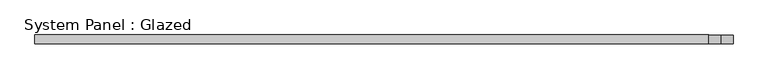
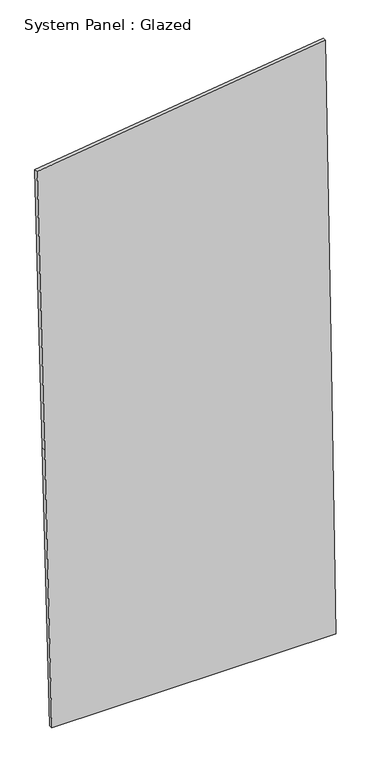
"""IFC4 building model written with IfcOpenShell, lengths in millimetres: plate geometry, System Panel : Glazed."""

from ifc_helpers import new_model, si_unit, frame, origin, place, context, project, spatial, polyline, outline, extrude, source, transform, mapped, element, save


def system_panel_glazed_6e61295c(model_context):
    return source(origin(), model_context, "Body", "SweptSolid", [
        extrude(outline(polyline([(0.0, -906.0305588), (0.0, 1006.3483292), (2123.3277595, 971.552521), (4246.6555191, 936.7567127), (3992.2264945, -1006.3483292), (1996.1132472, -956.189444), (0.0, -906.0305588)])), frame((0.0, -49.5, 0.0), z_axis=(0.0, 1.0, 0.0), x_axis=(0.0, 0.0, 1.0)), (0.0, 0.0, 1.0), 25.0),
    ])


if __name__ == "__main__":
    model = new_model("IFC4")
    model_context = context("Model", 3, world=origin())
    ifc_project = project(units=[si_unit("LENGTHUNIT", "METRE", prefix="MILLI")], contexts=[model_context])
    site = spatial("IfcSite", under=ifc_project)
    building = spatial("IfcBuilding", under=site)
    placement = place(None, origin())
    system_panel_glazed_shape = system_panel_glazed_6e61295c(model_context)
    element("IfcPlate", 1, ObjectType="System Panel : Glazed", at=placement, inside=building, context=model_context, shape_type="MappedRepresentation", body=[
        mapped(system_panel_glazed_shape, transform((0.0, 0.0, 0.0), x_axis=(1.0, 0.0, 0.0), y_axis=(0.0, 1.0, 0.0), z_axis=(0.0, 0.0, 1.0))),
    ])
    save(model, "model.ifc")

# Revit data of these elements
# Element 1 (IfcPlate, "System Panel : Glazed")
#   Materials on its faces: "Glass, Clear Glazing"
# Materials
#   "Glass, Clear Glazing": class "Glass", colour RGB 247 249 248, transparency 0.85, Description = "Clear glazing", Cost = 0
